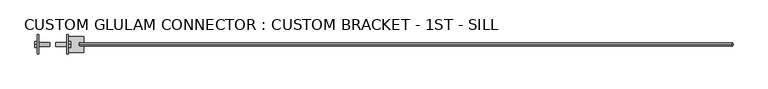
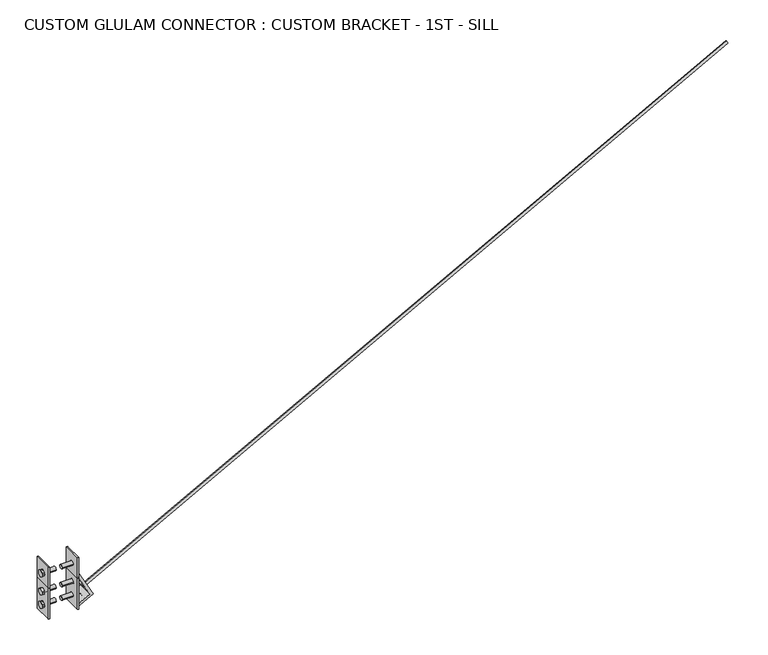
"""IFC4 building model written with IfcOpenShell, lengths in millimetres: fastener geometry, CUSTOM GLULAM CONNECTOR : CUSTOM BRACKET - 1ST - SILL."""

from ifc_helpers import new_model, si_unit, point, frame, frame_2d, origin, place, context, project, spatial, polyline, circle_curve, trimmed, segment, composite_curve, outline, extrude, source, transform, mapped, element, save
from ifc_brep_helpers import plane_surface, revolved_surface, advanced_brep


def custom_glulam_connector_custom_bracket_1st_sill_175718d5(model_context):
    return source(origin(), model_context, "Body", "SolidModel", [
        advanced_brep(
        [(-87.3125, 13.890625, 160.3375), (-95.25, 13.890625, 160.3375), (-95.25, -13.890625, 160.3375), (-87.3125, -13.890625, 160.3375), (-95.25, -60.325, 211.1375), (-95.25, -52.3875, 211.1375), (-95.25, 60.325, 211.1375), (-95.25, 60.325, 7.9375), (-95.25, -52.3875, 7.9375), (-95.25, -60.325, 7.9375), (-95.25, -13.890625, 71.4375), (-95.25, 13.890625, 71.4375), (-87.3125, 13.890625, 71.4375), (-87.3125, -13.890625, 71.4375), (-87.3125, -60.325, 211.1375), (-87.3125, -60.325, 7.9375), (-87.3125, 60.325, 7.9375), (-87.3125, 60.325, 211.1375)],
        [
            (0, 1),
            (1, 2, circle_curve(frame((-95.25, 0.0, 160.3375), z_axis=(-1.0, 0.0, 0.0), x_axis=(0.0, -1.0, 0.0)), 13.890625)),
            (2, 3),
            (3, 0, circle_curve(frame((-87.3125, 0.0, 160.3375), z_axis=(1.0, 0.0, 0.0), x_axis=(0.0, -1.0, 0.0)), 13.890625)),
            (4, 5),
            (5, 6),
            (6, 7),
            (7, 8),
            (8, 9),
            (9, 4),
            (1, 2, circle_curve(frame((-95.25, 0.0, 160.3375), z_axis=(1.0, 0.0, 0.0), x_axis=(0.0, -1.0, 0.0)), 13.890625)),
            (10, 11, circle_curve(frame((-95.25, 0.0, 71.4375), z_axis=(1.0, 0.0, 0.0), x_axis=(0.0, -1.0, 0.0)), 13.890625)),
            (11, 10, circle_curve(frame((-95.25, 0.0, 71.4375), z_axis=(1.0, 0.0, 0.0), x_axis=(0.0, -1.0, 0.0)), 13.890625)),
            (11, 12),
            (12, 13, circle_curve(frame((-87.3125, 0.0, 71.4375), z_axis=(1.0, 0.0, 0.0), x_axis=(0.0, -1.0, 0.0)), 13.890625)),
            (13, 10),
            (0, 3, circle_curve(frame((-87.3125, 0.0, 160.3375), z_axis=(1.0, 0.0, 0.0), x_axis=(0.0, -1.0, 0.0)), 13.890625)),
            (13, 12, circle_curve(frame((-87.3125, 0.0, 71.4375), z_axis=(1.0, 0.0, 0.0), x_axis=(0.0, -1.0, 0.0)), 13.890625)),
            (14, 15),
            (15, 16),
            (16, 17),
            (17, 14),
            (4, 14),
            (17, 6),
            (16, 7),
            (15, 9),
        ],
        [
            revolved_surface(polyline([(-95.25, -13.890625, 160.3375), (-87.3125, -13.890625, 160.3375)]), (-87.3125, 0.0, 160.3375), (-1.0, 0.0, 0.0)),
            plane_surface(frame((-95.25, 60.325, 211.1375), z_axis=(-1.0, 0.0, 0.0), x_axis=(0.0, 1.0, 0.0))),
            revolved_surface(polyline([(-95.25, -13.890625, 71.4375), (-87.3125, -13.890625, 71.4375)]), (-87.3125, 0.0, 71.4375), (-1.0, 0.0, 0.0)),
            plane_surface(frame((-87.3125, 60.325, 211.1375), z_axis=(1.0, 0.0, 0.0), x_axis=(0.0, -1.0, 0.0))),
            plane_surface(frame((-95.25, -60.325, 211.1375), z_axis=(0.0, 0.0, 1.0), x_axis=(1.0, 0.0, 0.0))),
            plane_surface(frame((-95.25, 60.325, 211.1375), z_axis=(0.0, 1.0, 0.0), x_axis=(1.0, 0.0, 0.0))),
            plane_surface(frame((-95.25, 60.325, 7.9375), z_axis=(0.0, 0.0, -1.0), x_axis=(1.0, 0.0, 0.0))),
            plane_surface(frame((-95.25, -60.325, 7.9375), z_axis=(0.0, -1.0, 0.0), x_axis=(1.0, 0.0, 0.0))),
        ],
        [
            (0, [[1, 2, 3, 4]]),
            (1, [[5, 6, 7, 8, 9, 10], [-2, 11], [12, 13]]),
            (2, [[14, 15, 16, -13]]),
            (0, [[-1, 17, -3, -11]]),
            (2, [[-14, -12, -16, 18]]),
            (3, [[19, 20, 21, 22], [-4, -17], [-18, -15]]),
            (4, [[-6, -5, 23, -22, 24]]),
            (5, [[-7, -24, -21, 25]]),
            (6, [[-9, -8, -25, -20, 26]]),
            (7, [[-10, -26, -19, -23]]),
        ],
    ),
        extrude(outline(polyline([(19.05, 171.3360226), (19.05, 149.3389774), (0.0, 138.3404547), (-19.05, 149.3389774), (-19.05, 171.3360226), (0.0, 182.3345453), (19.05, 171.3360226)])), frame((-110.2320312, 0.0, 0.0), z_axis=(1.0, 0.0, 0.0), x_axis=(0.0, 1.0, 0.0)), (0.0, 0.0, 1.0), 14.9820312),
        extrude(outline(composite_curve([segment(trimmed(circle_curve(frame_2d((0.0, 160.3375)), 12.7), [point((12.7, 160.3375))], [point((-12.7, 160.3375))], False, "CARTESIAN"), True, "CONTINUOUS"), segment(trimmed(circle_curve(frame_2d((0.0, 160.3375)), 12.7), [point((-12.7, 160.3375))], [point((12.7, 160.3375))], False, "CARTESIAN"), True, "CONTINUOUS")], self_intersect=False)), frame((-95.25, 0.0, 0.0), z_axis=(1.0, 0.0, 0.0), x_axis=(0.0, 1.0, 0.0)), (0.0, 0.0, 1.0), 76.2),
        extrude(outline(polyline([(19.05, 82.4360226), (19.05, 60.4389774), (0.0, 49.4404547), (-19.05, 60.4389774), (-19.05, 82.4360226), (0.0, 93.4345453), (19.05, 82.4360226)])), frame((-110.2320312, 0.0, 0.0), z_axis=(1.0, 0.0, 0.0), x_axis=(0.0, 1.0, 0.0)), (0.0, 0.0, 1.0), 14.9820312),
        extrude(outline(composite_curve([segment(trimmed(circle_curve(frame_2d((0.0, 71.4375)), 12.7), [point((12.7, 71.4375))], [point((-12.7, 71.4375))], False, "CARTESIAN"), True, "CONTINUOUS"), segment(trimmed(circle_curve(frame_2d((0.0, 71.4375)), 12.7), [point((-12.7, 71.4375))], [point((12.7, 71.4375))], False, "CARTESIAN"), True, "CONTINUOUS")], self_intersect=False)), frame((-95.25, 0.0, 0.0), z_axis=(1.0, 0.0, 0.0), x_axis=(0.0, 1.0, 0.0)), (0.0, 0.0, 1.0), 76.2),
        extrude(outline(polyline([(19.05, 171.3360226), (19.05, 149.3389774), (0.0, 138.3404547), (-19.05, 149.3389774), (-19.05, 171.3360226), (0.0, 182.3345453), (19.05, 171.3360226)])), frame((-110.2320312, 0.0, 0.0), z_axis=(1.0, 0.0, 0.0), x_axis=(0.0, 1.0, 0.0)), (0.0, 0.0, 1.0), 14.9820312),
        extrude(outline(composite_curve([segment(trimmed(circle_curve(frame_2d((0.0, 160.3375)), 12.7), [point((12.7, 160.3375))], [point((-12.7, 160.3375))], False, "CARTESIAN"), True, "CONTINUOUS"), segment(trimmed(circle_curve(frame_2d((0.0, 160.3375)), 12.7), [point((-12.7, 160.3375))], [point((12.7, 160.3375))], False, "CARTESIAN"), True, "CONTINUOUS")], self_intersect=False)), frame((-95.25, 0.0, 0.0), z_axis=(1.0, 0.0, 0.0), x_axis=(0.0, 1.0, 0.0)), (0.0, 0.0, 1.0), 76.2),
        advanced_brep(
        [(87.3125, 13.890625, 160.3375), (87.3125, -13.890625, 160.3375), (95.25, -13.890625, 160.3375), (95.25, 13.890625, 160.3375), (95.25, -60.325, 211.1375), (95.25, -60.325, 7.9375), (95.25, -52.3875, 7.9375), (95.25, 60.325, 7.9375), (95.25, 60.325, 211.1375), (95.25, -52.3875, 211.1375), (95.25, -13.890625, 71.4375), (95.25, 13.890625, 71.4375), (87.3125, -13.890625, 71.4375), (87.3125, 13.890625, 71.4375), (87.3125, -60.325, 211.1375), (87.3125, 60.325, 211.1375), (87.3125, 60.325, 7.9375), (87.3125, -60.325, 7.9375)],
        [
            (0, 1, circle_curve(frame((87.3125, 0.0, 160.3375), z_axis=(-1.0, 0.0, 0.0), x_axis=(0.0, -1.0, 0.0)), 13.890625)),
            (1, 2),
            (2, 3, circle_curve(frame((95.25, 0.0, 160.3375), z_axis=(1.0, 0.0, 0.0), x_axis=(0.0, -1.0, 0.0)), 13.890625)),
            (3, 0),
            (4, 5),
            (5, 6),
            (6, 7),
            (7, 8),
            (8, 9),
            (9, 4),
            (10, 11, circle_curve(frame((95.25, 0.0, 71.4375), z_axis=(-1.0, 0.0, 0.0), x_axis=(0.0, -1.0, 0.0)), 13.890625)),
            (11, 10, circle_curve(frame((95.25, 0.0, 71.4375), z_axis=(-1.0, 0.0, 0.0), x_axis=(0.0, -1.0, 0.0)), 13.890625)),
            (2, 3, circle_curve(frame((95.25, 0.0, 160.3375), z_axis=(-1.0, 0.0, 0.0), x_axis=(0.0, -1.0, 0.0)), 13.890625)),
            (10, 12),
            (12, 13, circle_curve(frame((87.3125, 0.0, 71.4375), z_axis=(-1.0, 0.0, 0.0), x_axis=(0.0, -1.0, 0.0)), 13.890625)),
            (13, 11),
            (1, 0, circle_curve(frame((87.3125, 0.0, 160.3375), z_axis=(-1.0, 0.0, 0.0), x_axis=(0.0, -1.0, 0.0)), 13.890625)),
            (13, 12, circle_curve(frame((87.3125, 0.0, 71.4375), z_axis=(-1.0, 0.0, 0.0), x_axis=(0.0, -1.0, 0.0)), 13.890625)),
            (14, 15),
            (15, 16),
            (16, 17),
            (17, 14),
            (8, 15),
            (14, 4),
            (7, 16),
            (5, 17),
        ],
        [
            revolved_surface(polyline([(95.25, -13.890625, 160.3375), (87.3125, -13.890625, 160.3375)]), (87.3125, 0.0, 160.3375), (1.0, 0.0, 0.0)),
            plane_surface(frame((95.25, 60.325, 211.1375), z_axis=(1.0, 0.0, 0.0), x_axis=(0.0, 1.0, 0.0))),
            revolved_surface(polyline([(95.25, -13.890625, 71.4375), (87.3125, -13.890625, 71.4375)]), (87.3125, 0.0, 71.4375), (1.0, 0.0, 0.0)),
            plane_surface(frame((87.3125, 60.325, 211.1375), z_axis=(-1.0, 0.0, 0.0), x_axis=(0.0, -1.0, 0.0))),
            plane_surface(frame((95.25, -60.325, 211.1375), z_axis=(0.0, 0.0, 1.0), x_axis=(-1.0, 0.0, 0.0))),
            plane_surface(frame((95.25, 60.325, 211.1375), z_axis=(0.0, 1.0, 0.0), x_axis=(-1.0, 0.0, 0.0))),
            plane_surface(frame((95.25, 60.325, 7.9375), z_axis=(0.0, 0.0, -1.0), x_axis=(-1.0, 0.0, 0.0))),
            plane_surface(frame((95.25, -60.325, 7.9375), z_axis=(0.0, -1.0, 0.0), x_axis=(-1.0, 0.0, 0.0))),
        ],
        [
            (0, [[1, 2, 3, 4]]),
            (1, [[5, 6, 7, 8, 9, 10], [11, 12], [13, -3]]),
            (2, [[-11, 14, 15, 16]]),
            (0, [[-13, -2, 17, -4]]),
            (2, [[18, -14, -12, -16]]),
            (3, [[19, 20, 21, 22], [-17, -1], [-15, -18]]),
            (4, [[23, -19, 24, -10, -9]]),
            (5, [[25, -20, -23, -8]]),
            (6, [[26, -21, -25, -7, -6]]),
            (7, [[-24, -22, -26, -5]]),
        ],
    ),
        extrude(outline(polyline([(19.05, 171.3360226), (19.05, 149.3389774), (0.0, 138.3404547), (-19.05, 149.3389774), (-19.05, 171.3360226), (0.0, 182.3345453), (19.05, 171.3360226)])), frame((95.25, 0.0, 0.0), z_axis=(1.0, 0.0, 0.0), x_axis=(0.0, 1.0, 0.0)), (0.0, 0.0, 1.0), 14.9820312),
        extrude(outline(composite_curve([segment(trimmed(circle_curve(frame_2d((0.0, 160.3375)), 12.7), [point((12.7, 160.3375))], [point((-12.7, 160.3375))], False, "CARTESIAN"), True, "CONTINUOUS"), segment(trimmed(circle_curve(frame_2d((0.0, 160.3375)), 12.7), [point((-12.7, 160.3375))], [point((12.7, 160.3375))], False, "CARTESIAN"), True, "CONTINUOUS")], self_intersect=False)), frame((19.05, 0.0, 0.0), z_axis=(1.0, 0.0, 0.0), x_axis=(0.0, 1.0, 0.0)), (0.0, 0.0, 1.0), 76.2),
        extrude(outline(polyline([(19.05, 82.4360226), (19.05, 60.4389774), (0.0, 49.4404547), (-19.05, 60.4389774), (-19.05, 82.4360226), (0.0, 93.4345453), (19.05, 82.4360226)])), frame((95.25, 0.0, 0.0), z_axis=(1.0, 0.0, 0.0), x_axis=(0.0, 1.0, 0.0)), (0.0, 0.0, 1.0), 14.9820312),
        extrude(outline(composite_curve([segment(trimmed(circle_curve(frame_2d((0.0, 71.4375)), 12.7), [point((12.7, 71.4375))], [point((-12.7, 71.4375))], False, "CARTESIAN"), True, "CONTINUOUS"), segment(trimmed(circle_curve(frame_2d((0.0, 71.4375)), 12.7), [point((-12.7, 71.4375))], [point((12.7, 71.4375))], False, "CARTESIAN"), True, "CONTINUOUS")], self_intersect=False)), frame((19.05, 0.0, 0.0), z_axis=(1.0, 0.0, 0.0), x_axis=(0.0, 1.0, 0.0)), (0.0, 0.0, 1.0), 76.2),
        extrude(outline(polyline([(19.05, 171.3360226), (19.05, 149.3389774), (0.0, 138.3404547), (-19.05, 149.3389774), (-19.05, 171.3360226), (0.0, 182.3345453), (19.05, 171.3360226)])), frame((95.25, 0.0, 0.0), z_axis=(1.0, 0.0, 0.0), x_axis=(0.0, 1.0, 0.0)), (0.0, 0.0, 1.0), 14.9820312),
        extrude(outline(composite_curve([segment(trimmed(circle_curve(frame_2d((0.0, 160.3375)), 12.7), [point((12.7, 160.3375))], [point((-12.7, 160.3375))], False, "CARTESIAN"), True, "CONTINUOUS"), segment(trimmed(circle_curve(frame_2d((0.0, 160.3375)), 12.7), [point((-12.7, 160.3375))], [point((12.7, 160.3375))], False, "CARTESIAN"), True, "CONTINUOUS")], self_intersect=False)), frame((19.05, 0.0, 0.0), z_axis=(1.0, 0.0, 0.0), x_axis=(0.0, 1.0, 0.0)), (0.0, 0.0, 1.0), 76.2),
        advanced_brep(
        [(-95.25, -60.325, 350.8375), (-95.25, -60.325, 211.1375), (-87.3125, -60.325, 211.1375), (-87.3125, -60.325, 350.8375), (-87.3125, 13.890625, 280.9875), (-95.25, 13.890625, 280.9875), (-95.25, -13.890625, 280.9875), (-87.3125, -13.890625, 280.9875), (-95.25, 60.325, 350.8375), (-95.25, 52.3875, 350.8375), (-87.3125, 60.325, 350.8375), (-95.25, 60.325, 211.1375), (-95.25, 52.3875, 211.1375), (-87.3125, 60.325, 211.1375)],
        [
            (0, 1),
            (1, 2),
            (2, 3),
            (3, 0),
            (4, 5),
            (5, 6, circle_curve(frame((-95.25, 0.0, 280.9875), z_axis=(-1.0, 0.0, 0.0), x_axis=(0.0, -1.0, 0.0)), 13.890625)),
            (6, 7),
            (7, 4, circle_curve(frame((-87.3125, 0.0, 280.9875), z_axis=(1.0, 0.0, 0.0), x_axis=(0.0, -1.0, 0.0)), 13.890625)),
            (4, 7, circle_curve(frame((-87.3125, 0.0, 280.9875), z_axis=(1.0, 0.0, 0.0), x_axis=(0.0, -1.0, 0.0)), 13.890625)),
            (6, 5, circle_curve(frame((-95.25, 0.0, 280.9875), z_axis=(-1.0, 0.0, 0.0), x_axis=(0.0, -1.0, 0.0)), 13.890625)),
            (8, 9),
            (9, 0),
            (3, 10),
            (10, 8),
            (8, 11),
            (11, 12),
            (12, 1),
            (2, 13),
            (13, 10),
            (13, 11),
        ],
        [
            plane_surface(frame((-95.25, -60.325, 211.1375), z_axis=(0.0, -1.0, 0.0), x_axis=(1.0, 0.0, 0.0))),
            revolved_surface(polyline([(-95.25, -13.890625, 280.9875), (-87.3125, -13.890625, 280.9875)]), (-87.3125, 0.0, 280.9875), (-1.0, 0.0, 0.0)),
            plane_surface(frame((-95.25, -60.325, 350.8375), z_axis=(0.0, 0.0, 1.0), x_axis=(1.0, 0.0, 0.0))),
            plane_surface(frame((-95.25, 60.325, 350.8375), z_axis=(-1.0, 0.0, 0.0), x_axis=(0.0, 1.0, 0.0))),
            plane_surface(frame((-87.3125, 60.325, 350.8375), z_axis=(1.0, 0.0, 0.0), x_axis=(0.0, -1.0, 0.0))),
            plane_surface(frame((-95.25, 60.325, 350.8375), z_axis=(0.0, 1.0, 0.0), x_axis=(1.0, 0.0, 0.0))),
            plane_surface(frame((-95.25, 60.325, 211.1375), z_axis=(0.0, 0.0, -1.0), x_axis=(1.0, 0.0, 0.0))),
        ],
        [
            (0, [[1, 2, 3, 4]]),
            (1, [[5, 6, 7, 8]]),
            (1, [[-5, 9, -7, 10]]),
            (2, [[11, 12, -4, 13, 14]]),
            (3, [[-12, -11, 15, 16, 17, -1], [-6, -10]]),
            (4, [[-3, 18, 19, -13], [-8, -9]]),
            (5, [[-15, -14, -19, 20]]),
            (6, [[-17, -16, -20, -18, -2]]),
        ],
    ),
        extrude(outline(polyline([(19.05, 291.9860226), (19.05, 269.9889774), (0.0, 258.9904547), (-19.05, 269.9889774), (-19.05, 291.9860226), (0.0, 302.9845453), (19.05, 291.9860226)])), frame((-110.2320312, 0.0, 0.0), z_axis=(1.0, 0.0, 0.0), x_axis=(0.0, 1.0, 0.0)), (0.0, 0.0, 1.0), 14.9820312),
        extrude(outline(composite_curve([segment(trimmed(circle_curve(frame_2d((0.0, 280.9875)), 12.7), [point((12.7, 280.9875))], [point((-12.7, 280.9875))], False, "CARTESIAN"), True, "CONTINUOUS"), segment(trimmed(circle_curve(frame_2d((0.0, 280.9875)), 12.7), [point((-12.7, 280.9875))], [point((12.7, 280.9875))], False, "CARTESIAN"), True, "CONTINUOUS")], self_intersect=False)), frame((-95.25, 0.0, 0.0), z_axis=(1.0, 0.0, 0.0), x_axis=(0.0, 1.0, 0.0)), (0.0, 0.0, 1.0), 76.2),
        advanced_brep(
        [(95.25, -60.325, 350.8375), (87.3125, -60.325, 350.8375), (87.3125, -60.325, 211.1375), (95.25, -60.325, 211.1375), (87.3125, 13.890625, 280.9875), (87.3125, -13.890625, 280.9875), (95.25, -13.890625, 280.9875), (95.25, 13.890625, 280.9875), (95.25, 60.325, 350.8375), (87.3125, 60.325, 350.8375), (95.25, 52.3875, 350.8375), (95.25, 52.3875, 211.1375), (95.25, 60.325, 211.1375), (87.3125, 60.325, 211.1375)],
        [
            (0, 1),
            (1, 2),
            (2, 3),
            (3, 0),
            (4, 5, circle_curve(frame((87.3125, 0.0, 280.9875), z_axis=(-1.0, 0.0, 0.0), x_axis=(0.0, -1.0, 0.0)), 13.890625)),
            (5, 6),
            (6, 7, circle_curve(frame((95.25, 0.0, 280.9875), z_axis=(1.0, 0.0, 0.0), x_axis=(0.0, -1.0, 0.0)), 13.890625)),
            (7, 4),
            (7, 6, circle_curve(frame((95.25, 0.0, 280.9875), z_axis=(1.0, 0.0, 0.0), x_axis=(0.0, -1.0, 0.0)), 13.890625)),
            (5, 4, circle_curve(frame((87.3125, 0.0, 280.9875), z_axis=(-1.0, 0.0, 0.0), x_axis=(0.0, -1.0, 0.0)), 13.890625)),
            (8, 9),
            (9, 1),
            (0, 10),
            (10, 8),
            (3, 11),
            (11, 12),
            (12, 8),
            (9, 13),
            (13, 2),
            (12, 13),
        ],
        [
            plane_surface(frame((95.25, -60.325, 211.1375), z_axis=(0.0, -1.0, 0.0), x_axis=(-1.0, 0.0, 0.0))),
            revolved_surface(polyline([(95.25, -13.890625, 280.9875), (87.3125, -13.890625, 280.9875)]), (87.3125, 0.0, 280.9875), (1.0, 0.0, 0.0)),
            plane_surface(frame((95.25, -60.325, 350.8375), z_axis=(0.0, 0.0, 1.0), x_axis=(-1.0, 0.0, 0.0))),
            plane_surface(frame((95.25, 60.325, 350.8375), z_axis=(1.0, 0.0, 0.0), x_axis=(0.0, 1.0, 0.0))),
            plane_surface(frame((87.3125, 60.325, 350.8375), z_axis=(-1.0, 0.0, 0.0), x_axis=(0.0, -1.0, 0.0))),
            plane_surface(frame((95.25, 60.325, 350.8375), z_axis=(0.0, 1.0, 0.0), x_axis=(-1.0, 0.0, 0.0))),
            plane_surface(frame((95.25, 60.325, 211.1375), z_axis=(0.0, 0.0, -1.0), x_axis=(-1.0, 0.0, 0.0))),
        ],
        [
            (0, [[1, 2, 3, 4]]),
            (1, [[5, 6, 7, 8]]),
            (1, [[9, -6, 10, -8]]),
            (2, [[11, 12, -1, 13, 14]]),
            (3, [[-4, 15, 16, 17, -14, -13], [-9, -7]]),
            (4, [[-12, 18, 19, -2], [-10, -5]]),
            (5, [[20, -18, -11, -17]]),
            (6, [[-3, -19, -20, -16, -15]]),
        ],
    ),
        extrude(outline(polyline([(19.05, 291.9860226), (19.05, 269.9889774), (0.0, 258.9904547), (-19.05, 269.9889774), (-19.05, 291.9860226), (0.0, 302.9845453), (19.05, 291.9860226)])), frame((95.25, 0.0, 0.0), z_axis=(1.0, 0.0, 0.0), x_axis=(0.0, 1.0, 0.0)), (0.0, 0.0, 1.0), 14.9820312),
        extrude(outline(composite_curve([segment(trimmed(circle_curve(frame_2d((0.0, 280.9875)), 12.7), [point((12.7, 280.9875))], [point((-12.7, 280.9875))], False, "CARTESIAN"), True, "CONTINUOUS"), segment(trimmed(circle_curve(frame_2d((0.0, 280.9875)), 12.7), [point((-12.7, 280.9875))], [point((12.7, 280.9875))], False, "CARTESIAN"), True, "CONTINUOUS")], self_intersect=False)), frame((19.05, 0.0, 0.0), z_axis=(1.0, 0.0, 0.0), x_axis=(0.0, 1.0, 0.0)), (0.0, 0.0, 1.0), 76.2),
        extrude(outline(composite_curve([segment(trimmed(circle_curve(frame_2d((0.0, 9.525)), 9.525), [point((0.0, 19.05))], [point((0.0, 0.0))], False, "CARTESIAN"), True, "CONTINUOUS"), segment(trimmed(circle_curve(frame_2d((0.0, 9.525)), 9.525), [point((0.0, 0.0))], [point((0.0, 19.05))], False, "CARTESIAN"), True, "CONTINUOUS")], self_intersect=False)), frame((173.2138238, 0.0, 105.1724436), z_axis=(0.8788171126619665, 0.0, 0.4771587602596065), x_axis=(0.0, 1.0, 0.0)), (0.0, 0.0, 1.0), 4597.4),
        advanced_brep(
        [(192.9085516, 50.8, 68.8992672), (95.25, 50.8, 15.875), (95.25, 50.8, 33.9390543), (171.3824347, 50.8, 75.2755936), (95.25, 50.8, 215.4940952), (95.25, 50.8, 248.7639444), (192.9085516, -50.8, 68.8992672), (95.25, -50.8, 248.7639444), (95.25, -50.8, 215.4940952), (171.3824347, -50.8, 75.2755936), (95.25, -50.8, 33.9390543), (95.25, -50.8, 15.875), (173.781941, 0.0, 104.1261019), (163.5558323, 0.0, 122.9602512), (149.6046106, 0.0, 115.3853559), (159.8307193, 0.0, 96.5512066), (141.0385275, 0.0, 58.8001963), (140.3409665, 0.0, 58.4214515), (147.9158618, 0.0, 44.4702298), (148.6134229, 0.0, 44.8489746)],
        [
            (0, 1),
            (1, 2),
            (2, 3),
            (3, 4),
            (4, 5),
            (5, 0),
            (6, 7),
            (7, 8),
            (8, 9),
            (9, 10),
            (10, 11),
            (11, 6),
            (5, 7),
            (6, 0),
            (12, 13, circle_curve(frame((168.6688866, 0.0, 113.5431766), z_axis=(-0.8788171126619665, 0.0, -0.4771587602596065), x_axis=(-0.4771587602596065, 0.0, 0.8788171126619665)), 10.715625)),
            (13, 12, circle_curve(frame((168.6688866, 0.0, 113.5431766), z_axis=(-0.8788171126619665, 0.0, -0.4771587602596065), x_axis=(-0.4771587602596065, 0.0, 0.8788171126619665)), 10.715625)),
            (4, 8),
            (3, 9),
            (14, 15, circle_curve(frame((154.717665, 0.0, 105.9682812), z_axis=(0.8788171126619665, 0.0, 0.4771587602596065), x_axis=(-0.4771587602596065, 0.0, 0.8788171126619665)), 10.715625)),
            (15, 14, circle_curve(frame((154.717665, 0.0, 105.9682812), z_axis=(0.8788171126619665, 0.0, 0.4771587602596065), x_axis=(-0.4771587602596065, 0.0, 0.8788171126619665)), 10.715625)),
            (2, 10),
            (16, 17, circle_curve(frame((140.689747, 0.0, 58.6108239), z_axis=(0.47715876025960524, 0.0, -0.8788171126619673), x_axis=(0.878817112661967, 0.0, 0.47715876025960513)), 0.396875)),
            (17, 16, circle_curve(frame((140.689747, 0.0, 58.6108239), z_axis=(0.47715876025960524, 0.0, -0.8788171126619673), x_axis=(0.878817112661967, 0.0, 0.47715876025960513)), 0.396875)),
            (1, 11),
            (18, 19, circle_curve(frame((148.2646423, 0.0, 44.6596022), z_axis=(-0.47715876025960524, 0.0, 0.8788171126619673), x_axis=(0.878817112661967, 0.0, 0.47715876025960513)), 0.396875)),
            (19, 18, circle_curve(frame((148.2646423, 0.0, 44.6596022), z_axis=(-0.47715876025960524, 0.0, 0.8788171126619673), x_axis=(0.878817112661967, 0.0, 0.47715876025960513)), 0.396875)),
            (13, 14),
            (15, 12),
            (19, 16),
            (17, 18),
        ],
        [
            plane_surface(frame((95.25, 50.8, 248.7639444), z_axis=(0.0, 1.0000000000000002, 0.0), x_axis=(-0.4771587602596065, 0.0, 0.8788171126619665))),
            plane_surface(frame((95.25, -50.8, 248.7639444), z_axis=(0.0, -1.0000000000000002, 0.0), x_axis=(0.4771587602596065, 0.0, -0.8788171126619665))),
            plane_surface(frame((192.9085516, 50.8, 68.8992672), z_axis=(0.8788171126619665, 0.0, 0.4771587602596065), x_axis=(0.0, -1.0, 0.0))),
            plane_surface(frame((95.25, 50.8, 248.7639444), z_axis=(-1.0, 0.0, 0.0), x_axis=(0.0, -1.0, 0.0))),
            plane_surface(frame((95.25, 50.8, 215.4940952), z_axis=(-0.8788171126619664, 0.0, -0.4771587602596066), x_axis=(0.0, -1.0, 0.0))),
            plane_surface(frame((171.3824347, 50.8, 75.2755936), z_axis=(-0.4771587602596049, 0.0, 0.8788171126619674), x_axis=(0.0, -1.0, 0.0))),
            plane_surface(frame((95.25, 50.8, 33.9390543), z_axis=(-1.0, 0.0, 0.0), x_axis=(0.0, -1.0, 0.0))),
            plane_surface(frame((95.25, 50.8, 15.875), z_axis=(0.4771587602596052, 0.0, -0.8788171126619672), x_axis=(0.0, -1.0, 0.0))),
            revolved_surface(polyline([(149.60461058960067, 0.0, 115.38535590022673), (163.55583228121063, 0.0, 122.9602512346057)]), (168.6688866, 0.0, 113.5431766), (-0.8788171126619665, 0.0, -0.4771587602596065)),
            revolved_surface(polyline([(141.0385274949113, 0.0, 58.80019629723707), (148.61342285819435, 0.0, 44.848974552392434)]), (148.2646423, 0.0, 44.6596022), (-0.47715876025960513, 0.0, 0.878817112661967)),
        ],
        [
            (0, [[1, 2, 3, 4, 5, 6]]),
            (1, [[7, 8, 9, 10, 11, 12]]),
            (2, [[13, -7, 14, -6], [15, 16]]),
            (3, [[17, -8, -13, -5]]),
            (4, [[18, -9, -17, -4], [19, 20]]),
            (5, [[21, -10, -18, -3], [22, 23]]),
            (6, [[24, -11, -21, -2]]),
            (7, [[-14, -12, -24, -1], [25, 26]]),
            (8, [[-16, 27, -20, 28]]),
            (8, [[-19, -27, -15, -28]]),
            (9, [[-26, 29, -23, 30]]),
            (9, [[-22, -29, -25, -30]]),
        ],
    ),
    ])


if __name__ == "__main__":
    model = new_model("IFC4")
    model_context = context("Model", 3, world=origin())
    ifc_project = project(units=[si_unit("LENGTHUNIT", "METRE", prefix="MILLI")], contexts=[model_context])
    site = spatial("IfcSite", under=ifc_project)
    building = spatial("IfcBuilding", under=site)
    placement = place(None, origin())
    custom_glulam_connector_custom_bracket_1st_sill_shape = custom_glulam_connector_custom_bracket_1st_sill_175718d5(model_context)
    element("IfcFastener", 1, ObjectType="CUSTOM GLULAM CONNECTOR : CUSTOM BRACKET - 1ST - SILL", at=placement, inside=building, context=model_context, shape_type="MappedRepresentation", body=[
        mapped(custom_glulam_connector_custom_bracket_1st_sill_shape, transform((0.0, 0.0, 0.0), x_axis=(1.0, 0.0, 0.0), y_axis=(0.0, 1.0, 0.0), z_axis=(0.0, 0.0, 1.0))),
    ])
    save(model, "model.ifc")

# Revit data of these elements
# Type "CUSTOM GLULAM CONNECTOR : CUSTOM BRACKET - 1ST - SILL"
#   Width - Top = 0' - 6 7/8"
#   Top/Bottom Plate Thickness = 0' - 0 5/16"
#   Top/Bottom Plate - Width = 0' - 7 1/2"
#   Rod Radius = 0' - 0 3/8"
#   Rod Length [instance default] = 1' - 0"
#   Plate Thickness = 0' - 0 5/16"
#   Offset - Upper Plate 2 = 0' - 0"
#   Height of Plate = 0' - 8"
#   Width - Bottom = 0' - 6 7/8"
#   Plate Width = 0' - 4 3/4"
#   Bracket Width = 0' - 4"
#   Bracket Thickness = 0' - 0 5/8"
#   Bracket Offset in X = 0' - 3 3/4"
#   Bracket Offset in Y = 0' - 0 3/8"
#   Bracket Offset = 0' - 0 5/8"
#   Bracket Leg = 0' - 4 3/8"
#   Bracket Hole Radius - Up = 0' - 0 27/64"
#   Bracket Hole Radius - Down = 0' - 0 1/64"
#   Bracket Hole Offset = 0' - 2"
#   Beam Width = 0' - 7 3/8"
#   Angle 2 = 28.50°
#   Angle 1 = 118.50°
#   Top Plate Visible = no
#   Rod Visibility = yes
#   Plate Visibility - Upper Right 2 = no
#   Plate Visibility - Upper Right 1 = yes
#   Plate Visibility - Upper Left 2 = no
#   Plate Visibility - Upper Left 1 = yes
#   Plate Visibility - Lower Right 2 = no
#   Plate Visibility - Lower Right 1 = yes
#   Plate Visibility - Lower Left 2 = no
#   Plate Visibility - Lower Left 1 = yes
#   Bracket Visibility = yes
#   Bottom Plate Visible = no
#   Upper Plates - 2 = element 1323965
#   Upper Plates - 1 = element 1323965
#   Lower Plates = element 1339837
#   Bracket Material = 5/8" STEEL ANGLE (HDG AFTER FABRICATION)
#   URL = ""
# Element 1 (IfcFastener, "CUSTOM GLULAM CONNECTOR : CUSTOM BRACKET - 1ST - SILL")
#   Rod Length = 15' - 1"
#   Materials on its faces: "1\" GALV. LAG BOLT (LENGTH = 1/2\" SHY OF GLULAM DEPTH) -  (GALV. THRU BOLT IF PLATE ON OPP. SIDE OF STRUCT MEMBER)", "5/16\" STEEL PLATE (HDG AFTER FABRICATION)", "5/8\" STEEL ANGLE (HDG AFTER FABRICATION)", "3/4\" GALV. ROD (THREADED AT ENDS) - TURN BUCKLE AT 1/4 POINT OF TOTAL LENGTH"
# Materials
#   "5/8\" STEEL ANGLE (HDG AFTER FABRICATION)": class "Generic", colour RGB 195 195 195, transparency 0, Cost = 0
#   "1\" GALV. LAG BOLT (LENGTH = 1/2\" SHY OF GLULAM DEPTH) -  (GALV. THRU BOLT IF PLATE ON OPP. SIDE OF STRUCT MEMBER)": class "Generic", colour RGB 120 120 120, transparency 0, Cost = 0
#   "5/16\" STEEL PLATE (HDG AFTER FABRICATION)": class "Generic", colour RGB 232 232 232, transparency 0, Cost = 0
#   "3/4\" GALV. ROD (THREADED AT ENDS) - TURN BUCKLE AT 1/4 POINT OF TOTAL LENGTH": class "Generic", colour RGB 120 120 120, transparency 0, Cost = 0
